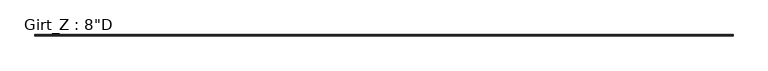
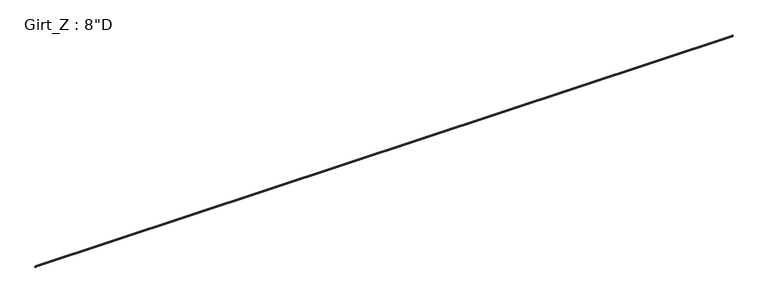
"""IFC4 building model written with IfcOpenShell, lengths in millimetres: beam geometry."""

from ifc_helpers import new_model, si_unit, point, frame, frame_2d, origin, place, context, project, spatial, polyline, circle_curve, trimmed, segment, composite_curve, outline, extrude, source, transform, mapped, element, save


def beam_38e0474f(model_context):
    return source(origin(), model_context, "Body", "SweptSolid", [
        extrude(outline(composite_curve([segment(polyline([(-63.5, 101.6), (-3.3734375, 101.6)]), True, "CONTINUOUS"), segment(trimmed(circle_curve(frame_2d((-3.3734375, 96.8375)), 4.7625), [point((-3.3734375, 101.6))], [point((1.3890625, 96.8375))], False, "CARTESIAN"), True, "CONTINUOUS"), segment(polyline([(1.3890625, 96.8375), (1.3890625, -96.8389339)]), True, "CONTINUOUS"), segment(trimmed(circle_curve(frame_2d((3.3748024, -96.8389339)), 1.9857399), [point((1.3890625, -96.8389339))], [point((3.2694106, -98.821875))], True, "CARTESIAN"), True, "CONTINUOUS"), segment(polyline([(3.2694106, -98.821875), (62.204539, -98.821875), (73.6169367, -85.221109), (75.745104, -87.0068534), (63.5, -101.6), (3.3734375, -101.6)]), True, "CONTINUOUS"), segment(trimmed(circle_curve(frame_2d((3.3734375, -96.8375)), 4.7625), [point((3.3734375, -101.6))], [point((-1.3890625, -96.8375))], False, "CARTESIAN"), True, "CONTINUOUS"), segment(polyline([(-1.3890625, -96.8375), (-1.3890625, 96.8381931)]), True, "CONTINUOUS"), segment(trimmed(circle_curve(frame_2d((-3.3741066, 96.8381931)), 1.9850441), [point((-1.3890625, 96.8381931))], [point((-3.3005807, 98.821875))], True, "CARTESIAN"), True, "CONTINUOUS"), segment(polyline([(-3.3005807, 98.821875), (-62.204539, 98.821875), (-73.6169367, 85.221109), (-75.745104, 87.0068534), (-63.5, 101.6)]), True, "CONTINUOUS")], self_intersect=False)), frame((-40666.0697266, 0.0, 0.0), z_axis=(1.0, 0.0, 0.0), x_axis=(0.0, 1.0, 0.0)), (0.0, 0.0, 1.0), 81171.8019531),
    ])


if __name__ == "__main__":
    model = new_model("IFC4")
    model_context = context("Model", 3, world=origin())
    ifc_project = project(units=[si_unit("LENGTHUNIT", "METRE", prefix="MILLI")], contexts=[model_context])
    site = spatial("IfcSite", under=ifc_project)
    building = spatial("IfcBuilding", under=site)
    placement = place(None, origin())
    beam_shape = beam_38e0474f(model_context)
    element("IfcBeam", 1, ObjectType="Girt_Z : 8\"D", at=placement, inside=building, context=model_context, shape_type="MappedRepresentation", body=[
        mapped(beam_shape, transform((0.0, 0.0, 0.0), x_axis=(1.0, 0.0, 0.0), y_axis=(0.0, 1.0, 0.0), z_axis=(0.0, 0.0, 1.0))),
    ])
    save(model, "model.ifc")

# Revit data of these elements
# Type "Girt_Z : 8\"D"
#   Web_Thickness = 0' - 0 7/64"
#   Length [instance default] = 10' - 0"
#   Leg_1 = 0' - 2 1/2"
#   Height = 0' - 8"
#   Structural Material [instance default] = none
# Element 1 (IfcBeam, "Girt_Z : 8\"D")
#   Structural Material = Steel
#   Materials on its faces: "Steel"
# Materials
#   "Steel": class "Metal", colour RGB 118 118 114, transparency 0, Description = "Steel, mill finish", Cost = 0
